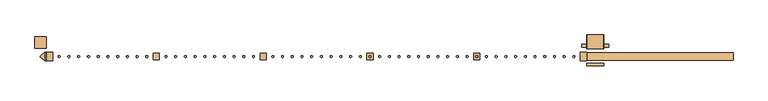
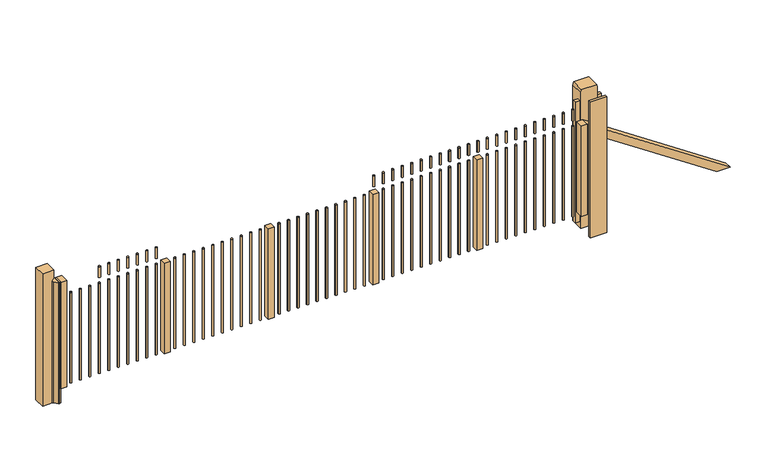
"""IFC4 building model written with IfcOpenShell, lengths in millimetres: door geometry, NLRS_90_DO_UN_schuifpoort met spijlen_gen_rsf : schuifpoort automatisch bxh 7000x1800-NP."""

from ifc_helpers import new_model, si_unit, point, frame, frame_2d, origin, place, context, project, spatial, polyline, circle_curve, trimmed, segment, composite_curve, outline, extrude, source, transform, mapped, element, save


def door_7189267d(model_context):
    return source(origin(), model_context, "Body", "SweptSolid", [
        extrude(outline(composite_curve([segment(trimmed(circle_curve(frame_2d((3299.5, 0.0)), 12.5), [point((3312.0, 0.0))], [point((3287.0, 0.0))], False, "CARTESIAN"), True, "CONTINUOUS"), segment(trimmed(circle_curve(frame_2d((3299.5, 0.0)), 12.5), [point((3287.0, 0.0))], [point((3312.0, 0.0))], False, "CARTESIAN"), True, "CONTINUOUS")], self_intersect=False)), frame((0.0, 0.0, 300.0), z_axis=(0.0, 0.0, 1.0), x_axis=(1.0, 0.0, 0.0)), (0.0, 0.0, 1.0), 1270.0),
        extrude(outline(composite_curve([segment(trimmed(circle_curve(frame_2d((3173.5, 0.0)), 12.5), [point((3186.0, 0.0))], [point((3161.0, 0.0))], False, "CARTESIAN"), True, "CONTINUOUS"), segment(trimmed(circle_curve(frame_2d((3173.5, 0.0)), 12.5), [point((3161.0, 0.0))], [point((3186.0, 0.0))], False, "CARTESIAN"), True, "CONTINUOUS")], self_intersect=False)), frame((0.0, 0.0, 300.0), z_axis=(0.0, 0.0, 1.0), x_axis=(1.0, 0.0, 0.0)), (0.0, 0.0, 1.0), 1270.0),
        extrude(outline(composite_curve([segment(trimmed(circle_curve(frame_2d((3047.5, 0.0)), 12.5), [point((3060.0, 0.0))], [point((3035.0, 0.0))], False, "CARTESIAN"), True, "CONTINUOUS"), segment(trimmed(circle_curve(frame_2d((3047.5, 0.0)), 12.5), [point((3035.0, 0.0))], [point((3060.0, 0.0))], False, "CARTESIAN"), True, "CONTINUOUS")], self_intersect=False)), frame((0.0, 0.0, 300.0), z_axis=(0.0, 0.0, 1.0), x_axis=(1.0, 0.0, 0.0)), (0.0, 0.0, 1.0), 1270.0),
        extrude(outline(composite_curve([segment(trimmed(circle_curve(frame_2d((2921.5, 0.0)), 12.5), [point((2934.0, 0.0))], [point((2909.0, 0.0))], False, "CARTESIAN"), True, "CONTINUOUS"), segment(trimmed(circle_curve(frame_2d((2921.5, 0.0)), 12.5), [point((2909.0, 0.0))], [point((2934.0, 0.0))], False, "CARTESIAN"), True, "CONTINUOUS")], self_intersect=False)), frame((0.0, 0.0, 300.0), z_axis=(0.0, 0.0, 1.0), x_axis=(1.0, 0.0, 0.0)), (0.0, 0.0, 1.0), 1270.0),
        extrude(outline(composite_curve([segment(trimmed(circle_curve(frame_2d((2795.5, 0.0)), 12.5), [point((2808.0, 0.0))], [point((2783.0, 0.0))], False, "CARTESIAN"), True, "CONTINUOUS"), segment(trimmed(circle_curve(frame_2d((2795.5, 0.0)), 12.5), [point((2783.0, 0.0))], [point((2808.0, 0.0))], False, "CARTESIAN"), True, "CONTINUOUS")], self_intersect=False)), frame((0.0, 0.0, 300.0), z_axis=(0.0, 0.0, 1.0), x_axis=(1.0, 0.0, 0.0)), (0.0, 0.0, 1.0), 1270.0),
        extrude(outline(composite_curve([segment(trimmed(circle_curve(frame_2d((2669.5, 0.0)), 12.5), [point((2682.0, 0.0))], [point((2657.0, 0.0))], False, "CARTESIAN"), True, "CONTINUOUS"), segment(trimmed(circle_curve(frame_2d((2669.5, 0.0)), 12.5), [point((2657.0, 0.0))], [point((2682.0, 0.0))], False, "CARTESIAN"), True, "CONTINUOUS")], self_intersect=False)), frame((0.0, 0.0, 300.0), z_axis=(0.0, 0.0, 1.0), x_axis=(1.0, 0.0, 0.0)), (0.0, 0.0, 1.0), 1270.0),
        extrude(outline(composite_curve([segment(trimmed(circle_curve(frame_2d((2543.5, 0.0)), 12.5), [point((2556.0, 0.0))], [point((2531.0, 0.0))], False, "CARTESIAN"), True, "CONTINUOUS"), segment(trimmed(circle_curve(frame_2d((2543.5, 0.0)), 12.5), [point((2531.0, 0.0))], [point((2556.0, 0.0))], False, "CARTESIAN"), True, "CONTINUOUS")], self_intersect=False)), frame((0.0, 0.0, 300.0), z_axis=(0.0, 0.0, 1.0), x_axis=(1.0, 0.0, 0.0)), (0.0, 0.0, 1.0), 1270.0),
        extrude(outline(composite_curve([segment(trimmed(circle_curve(frame_2d((2417.5, 0.0)), 12.5), [point((2430.0, 0.0))], [point((2405.0, 0.0))], False, "CARTESIAN"), True, "CONTINUOUS"), segment(trimmed(circle_curve(frame_2d((2417.5, 0.0)), 12.5), [point((2405.0, 0.0))], [point((2430.0, 0.0))], False, "CARTESIAN"), True, "CONTINUOUS")], self_intersect=False)), frame((0.0, 0.0, 300.0), z_axis=(0.0, 0.0, 1.0), x_axis=(1.0, 0.0, 0.0)), (0.0, 0.0, 1.0), 1270.0),
        extrude(outline(composite_curve([segment(trimmed(circle_curve(frame_2d((2291.5, 0.0)), 12.5), [point((2304.0, 0.0))], [point((2279.0, 0.0))], False, "CARTESIAN"), True, "CONTINUOUS"), segment(trimmed(circle_curve(frame_2d((2291.5, 0.0)), 12.5), [point((2279.0, 0.0))], [point((2304.0, 0.0))], False, "CARTESIAN"), True, "CONTINUOUS")], self_intersect=False)), frame((0.0, 0.0, 300.0), z_axis=(0.0, 0.0, 1.0), x_axis=(1.0, 0.0, 0.0)), (0.0, 0.0, 1.0), 1270.0),
        extrude(outline(composite_curve([segment(trimmed(circle_curve(frame_2d((2165.5, 0.0)), 12.5), [point((2178.0, 0.0))], [point((2153.0, 0.0))], False, "CARTESIAN"), True, "CONTINUOUS"), segment(trimmed(circle_curve(frame_2d((2165.5, 0.0)), 12.5), [point((2153.0, 0.0))], [point((2178.0, 0.0))], False, "CARTESIAN"), True, "CONTINUOUS")], self_intersect=False)), frame((0.0, 0.0, 300.0), z_axis=(0.0, 0.0, 1.0), x_axis=(1.0, 0.0, 0.0)), (0.0, 0.0, 1.0), 1270.0),
        extrude(outline(composite_curve([segment(trimmed(circle_curve(frame_2d((1915.5, 0.0)), 12.5), [point((1928.0, 0.0))], [point((1903.0, 0.0))], False, "CARTESIAN"), True, "CONTINUOUS"), segment(trimmed(circle_curve(frame_2d((1915.5, 0.0)), 12.5), [point((1903.0, 0.0))], [point((1928.0, 0.0))], False, "CARTESIAN"), True, "CONTINUOUS")], self_intersect=False)), frame((0.0, 0.0, 300.0), z_axis=(0.0, 0.0, 1.0), x_axis=(1.0, 0.0, 0.0)), (0.0, 0.0, 1.0), 1270.0),
        extrude(outline(composite_curve([segment(trimmed(circle_curve(frame_2d((1789.5, 0.0)), 12.5), [point((1802.0, 0.0))], [point((1777.0, 0.0))], False, "CARTESIAN"), True, "CONTINUOUS"), segment(trimmed(circle_curve(frame_2d((1789.5, 0.0)), 12.5), [point((1777.0, 0.0))], [point((1802.0, 0.0))], False, "CARTESIAN"), True, "CONTINUOUS")], self_intersect=False)), frame((0.0, 0.0, 300.0), z_axis=(0.0, 0.0, 1.0), x_axis=(1.0, 0.0, 0.0)), (0.0, 0.0, 1.0), 1270.0),
        extrude(outline(composite_curve([segment(trimmed(circle_curve(frame_2d((1663.5, 0.0)), 12.5), [point((1676.0, 0.0))], [point((1651.0, 0.0))], False, "CARTESIAN"), True, "CONTINUOUS"), segment(trimmed(circle_curve(frame_2d((1663.5, 0.0)), 12.5), [point((1651.0, 0.0))], [point((1676.0, 0.0))], False, "CARTESIAN"), True, "CONTINUOUS")], self_intersect=False)), frame((0.0, 0.0, 300.0), z_axis=(0.0, 0.0, 1.0), x_axis=(1.0, 0.0, 0.0)), (0.0, 0.0, 1.0), 1270.0),
        extrude(outline(composite_curve([segment(trimmed(circle_curve(frame_2d((1537.5, 0.0)), 12.5), [point((1550.0, 0.0))], [point((1525.0, 0.0))], False, "CARTESIAN"), True, "CONTINUOUS"), segment(trimmed(circle_curve(frame_2d((1537.5, 0.0)), 12.5), [point((1525.0, 0.0))], [point((1550.0, 0.0))], False, "CARTESIAN"), True, "CONTINUOUS")], self_intersect=False)), frame((0.0, 0.0, 300.0), z_axis=(0.0, 0.0, 1.0), x_axis=(1.0, 0.0, 0.0)), (0.0, 0.0, 1.0), 1270.0),
        extrude(outline(composite_curve([segment(trimmed(circle_curve(frame_2d((1411.5, 0.0)), 12.5), [point((1424.0, 0.0))], [point((1399.0, 0.0))], False, "CARTESIAN"), True, "CONTINUOUS"), segment(trimmed(circle_curve(frame_2d((1411.5, 0.0)), 12.5), [point((1399.0, 0.0))], [point((1424.0, 0.0))], False, "CARTESIAN"), True, "CONTINUOUS")], self_intersect=False)), frame((0.0, 0.0, 300.0), z_axis=(0.0, 0.0, 1.0), x_axis=(1.0, 0.0, 0.0)), (0.0, 0.0, 1.0), 1270.0),
        extrude(outline(composite_curve([segment(trimmed(circle_curve(frame_2d((1285.5, 0.0)), 12.5), [point((1298.0, 0.0))], [point((1273.0, 0.0))], False, "CARTESIAN"), True, "CONTINUOUS"), segment(trimmed(circle_curve(frame_2d((1285.5, 0.0)), 12.5), [point((1273.0, 0.0))], [point((1298.0, 0.0))], False, "CARTESIAN"), True, "CONTINUOUS")], self_intersect=False)), frame((0.0, 0.0, 300.0), z_axis=(0.0, 0.0, 1.0), x_axis=(1.0, 0.0, 0.0)), (0.0, 0.0, 1.0), 1270.0),
        extrude(outline(composite_curve([segment(trimmed(circle_curve(frame_2d((1159.5, 0.0)), 12.5), [point((1172.0, 0.0))], [point((1147.0, 0.0))], False, "CARTESIAN"), True, "CONTINUOUS"), segment(trimmed(circle_curve(frame_2d((1159.5, 0.0)), 12.5), [point((1147.0, 0.0))], [point((1172.0, 0.0))], False, "CARTESIAN"), True, "CONTINUOUS")], self_intersect=False)), frame((0.0, 0.0, 300.0), z_axis=(0.0, 0.0, 1.0), x_axis=(1.0, 0.0, 0.0)), (0.0, 0.0, 1.0), 1270.0),
        extrude(outline(composite_curve([segment(trimmed(circle_curve(frame_2d((1033.5, 0.0)), 12.5), [point((1046.0, 0.0))], [point((1021.0, 0.0))], False, "CARTESIAN"), True, "CONTINUOUS"), segment(trimmed(circle_curve(frame_2d((1033.5, 0.0)), 12.5), [point((1021.0, 0.0))], [point((1046.0, 0.0))], False, "CARTESIAN"), True, "CONTINUOUS")], self_intersect=False)), frame((0.0, 0.0, 300.0), z_axis=(0.0, 0.0, 1.0), x_axis=(1.0, 0.0, 0.0)), (0.0, 0.0, 1.0), 1270.0),
        extrude(outline(composite_curve([segment(trimmed(circle_curve(frame_2d((907.5, 0.0)), 12.5), [point((920.0, 0.0))], [point((895.0, 0.0))], False, "CARTESIAN"), True, "CONTINUOUS"), segment(trimmed(circle_curve(frame_2d((907.5, 0.0)), 12.5), [point((895.0, 0.0))], [point((920.0, 0.0))], False, "CARTESIAN"), True, "CONTINUOUS")], self_intersect=False)), frame((0.0, 0.0, 300.0), z_axis=(0.0, 0.0, 1.0), x_axis=(1.0, 0.0, 0.0)), (0.0, 0.0, 1.0), 1270.0),
        extrude(outline(composite_curve([segment(trimmed(circle_curve(frame_2d((781.5, 0.0)), 12.5), [point((794.0, 0.0))], [point((769.0, 0.0))], False, "CARTESIAN"), True, "CONTINUOUS"), segment(trimmed(circle_curve(frame_2d((781.5, 0.0)), 12.5), [point((769.0, 0.0))], [point((794.0, 0.0))], False, "CARTESIAN"), True, "CONTINUOUS")], self_intersect=False)), frame((0.0, 0.0, 300.0), z_axis=(0.0, 0.0, 1.0), x_axis=(1.0, 0.0, 0.0)), (0.0, 0.0, 1.0), 1270.0),
        extrude(outline(polyline([(3465.0, 158.5), (3465.0, 118.5), (3400.0, 118.5), (3400.0, 158.5), (3465.0, 158.5)])), frame((0.0, 0.0, 100.0), z_axis=(0.0, 0.0, 1.0), x_axis=(1.0, 0.0, 0.0)), (0.0, 0.0, 1.0), 1700.0),
        extrude(outline(polyline([(3685.0, 158.5), (3750.0, 158.5), (3750.0, 118.5), (3685.0, 118.5), (3685.0, 158.5)])), frame((0.0, 0.0, 100.0), z_axis=(0.0, 0.0, 1.0), x_axis=(1.0, 0.0, 0.0)), (0.0, 0.0, 1.0), 1700.0),
        extrude(outline(polyline([(3685.0, -84.5), (3685.0, -119.5), (3465.0, -119.5), (3465.0, -84.5), (3685.0, -84.5)])), frame((0.0, 0.0, 12.0), z_axis=(0.0, 0.0, 1.0), x_axis=(1.0, 0.0, 0.0)), (0.0, 0.0, 1.0), 1906.0),
        extrude(outline(polyline([(1918.0, 3465.0), (12.0, 3465.0), (12.0, 3685.0), (1918.0, 3685.0), (1960.0, 3677.5), (1960.0, 3472.5), (1918.0, 3465.0)])), frame((0.0, 100.5, 0.0), z_axis=(0.0, 1.0, 0.0), x_axis=(0.0, 0.0, 1.0)), (0.0, 0.0, 1.0), 180.0),
        extrude(outline(polyline([(2000.5, 40.0), (2080.5, 40.0), (2080.5, -40.0), (2000.5, -40.0), (2000.5, 40.0)])), frame((0.0, 0.0, 300.0), z_axis=(0.0, 0.0, 1.0), x_axis=(1.0, 0.0, 0.0)), (0.0, 0.0, 1.0), 1270.0),
        extrude(outline(polyline([(616.5, 40.0), (696.5, 40.0), (696.5, -40.0), (616.5, -40.0), (616.5, 40.0)])), frame((0.0, 0.0, 300.0), z_axis=(0.0, 0.0, 1.0), x_axis=(1.0, 0.0, 0.0)), (0.0, 0.0, 1.0), 1270.0),
        extrude(outline(polyline([(-767.5, 40.0), (-687.5, 40.0), (-687.5, -40.0), (-767.5, -40.0), (-767.5, 40.0)])), frame((0.0, 0.0, 300.0), z_axis=(0.0, 0.0, 1.0), x_axis=(1.0, 0.0, 0.0)), (0.0, 0.0, 1.0), 1270.0),
        extrude(outline(polyline([(-2151.5, 40.0), (-2071.5, 40.0), (-2071.5, -40.0), (-2151.5, -40.0), (-2151.5, 40.0)])), frame((0.0, 0.0, 300.0), z_axis=(0.0, 0.0, 1.0), x_axis=(1.0, 0.0, 0.0)), (0.0, 0.0, 1.0), 1270.0),
        extrude(outline(composite_curve([segment(trimmed(circle_curve(frame_2d((531.5, 0.0)), 12.5), [point((544.0, 0.0))], [point((519.0, 0.0))], False, "CARTESIAN"), True, "CONTINUOUS"), segment(trimmed(circle_curve(frame_2d((531.5, 0.0)), 12.5), [point((519.0, 0.0))], [point((544.0, 0.0))], False, "CARTESIAN"), True, "CONTINUOUS")], self_intersect=False)), frame((0.0, 0.0, 300.0), z_axis=(0.0, 0.0, 1.0), x_axis=(1.0, 0.0, 0.0)), (0.0, 0.0, 1.0), 1270.0),
        extrude(outline(composite_curve([segment(trimmed(circle_curve(frame_2d((405.5, 0.0)), 12.5), [point((418.0, 0.0))], [point((393.0, 0.0))], False, "CARTESIAN"), True, "CONTINUOUS"), segment(trimmed(circle_curve(frame_2d((405.5, 0.0)), 12.5), [point((393.0, 0.0))], [point((418.0, 0.0))], False, "CARTESIAN"), True, "CONTINUOUS")], self_intersect=False)), frame((0.0, 0.0, 300.0), z_axis=(0.0, 0.0, 1.0), x_axis=(1.0, 0.0, 0.0)), (0.0, 0.0, 1.0), 1270.0),
        extrude(outline(composite_curve([segment(trimmed(circle_curve(frame_2d((279.5, 0.0)), 12.5), [point((292.0, 0.0))], [point((267.0, 0.0))], False, "CARTESIAN"), True, "CONTINUOUS"), segment(trimmed(circle_curve(frame_2d((279.5, 0.0)), 12.5), [point((267.0, 0.0))], [point((292.0, 0.0))], False, "CARTESIAN"), True, "CONTINUOUS")], self_intersect=False)), frame((0.0, 0.0, 300.0), z_axis=(0.0, 0.0, 1.0), x_axis=(1.0, 0.0, 0.0)), (0.0, 0.0, 1.0), 1270.0),
        extrude(outline(composite_curve([segment(trimmed(circle_curve(frame_2d((153.5, 0.0)), 12.5), [point((166.0, 0.0))], [point((141.0, 0.0))], False, "CARTESIAN"), True, "CONTINUOUS"), segment(trimmed(circle_curve(frame_2d((153.5, 0.0)), 12.5), [point((141.0, 0.0))], [point((166.0, 0.0))], False, "CARTESIAN"), True, "CONTINUOUS")], self_intersect=False)), frame((0.0, 0.0, 300.0), z_axis=(0.0, 0.0, 1.0), x_axis=(1.0, 0.0, 0.0)), (0.0, 0.0, 1.0), 1270.0),
        extrude(outline(composite_curve([segment(trimmed(circle_curve(frame_2d((27.5, 0.0)), 12.5), [point((40.0, 0.0))], [point((15.0, 0.0))], False, "CARTESIAN"), True, "CONTINUOUS"), segment(trimmed(circle_curve(frame_2d((27.5, 0.0)), 12.5), [point((15.0, 0.0))], [point((40.0, 0.0))], False, "CARTESIAN"), True, "CONTINUOUS")], self_intersect=False)), frame((0.0, 0.0, 300.0), z_axis=(0.0, 0.0, 1.0), x_axis=(1.0, 0.0, 0.0)), (0.0, 0.0, 1.0), 1270.0),
        extrude(outline(composite_curve([segment(trimmed(circle_curve(frame_2d((-98.5, 0.0)), 12.5), [point((-86.0, 0.0))], [point((-111.0, 0.0))], False, "CARTESIAN"), True, "CONTINUOUS"), segment(trimmed(circle_curve(frame_2d((-98.5, 0.0)), 12.5), [point((-111.0, 0.0))], [point((-86.0, 0.0))], False, "CARTESIAN"), True, "CONTINUOUS")], self_intersect=False)), frame((0.0, 0.0, 300.0), z_axis=(0.0, 0.0, 1.0), x_axis=(1.0, 0.0, 0.0)), (0.0, 0.0, 1.0), 1270.0),
        extrude(outline(composite_curve([segment(trimmed(circle_curve(frame_2d((-224.5, 0.0)), 12.5), [point((-212.0, 0.0))], [point((-237.0, 0.0))], False, "CARTESIAN"), True, "CONTINUOUS"), segment(trimmed(circle_curve(frame_2d((-224.5, 0.0)), 12.5), [point((-237.0, 0.0))], [point((-212.0, 0.0))], False, "CARTESIAN"), True, "CONTINUOUS")], self_intersect=False)), frame((0.0, 0.0, 300.0), z_axis=(0.0, 0.0, 1.0), x_axis=(1.0, 0.0, 0.0)), (0.0, 0.0, 1.0), 1270.0),
        extrude(outline(composite_curve([segment(trimmed(circle_curve(frame_2d((-350.5, 0.0)), 12.5), [point((-338.0, 0.0))], [point((-363.0, 0.0))], False, "CARTESIAN"), True, "CONTINUOUS"), segment(trimmed(circle_curve(frame_2d((-350.5, 0.0)), 12.5), [point((-363.0, 0.0))], [point((-338.0, 0.0))], False, "CARTESIAN"), True, "CONTINUOUS")], self_intersect=False)), frame((0.0, 0.0, 300.0), z_axis=(0.0, 0.0, 1.0), x_axis=(1.0, 0.0, 0.0)), (0.0, 0.0, 1.0), 1270.0),
        extrude(outline(composite_curve([segment(trimmed(circle_curve(frame_2d((-476.5, 0.0)), 12.5), [point((-464.0, 0.0))], [point((-489.0, 0.0))], False, "CARTESIAN"), True, "CONTINUOUS"), segment(trimmed(circle_curve(frame_2d((-476.5, 0.0)), 12.5), [point((-489.0, 0.0))], [point((-464.0, 0.0))], False, "CARTESIAN"), True, "CONTINUOUS")], self_intersect=False)), frame((0.0, 0.0, 300.0), z_axis=(0.0, 0.0, 1.0), x_axis=(1.0, 0.0, 0.0)), (0.0, 0.0, 1.0), 1270.0),
        extrude(outline(composite_curve([segment(trimmed(circle_curve(frame_2d((-602.5, 0.0)), 12.5), [point((-590.0, 0.0))], [point((-615.0, 0.0))], False, "CARTESIAN"), True, "CONTINUOUS"), segment(trimmed(circle_curve(frame_2d((-602.5, 0.0)), 12.5), [point((-615.0, 0.0))], [point((-590.0, 0.0))], False, "CARTESIAN"), True, "CONTINUOUS")], self_intersect=False)), frame((0.0, 0.0, 300.0), z_axis=(0.0, 0.0, 1.0), x_axis=(1.0, 0.0, 0.0)), (0.0, 0.0, 1.0), 1270.0),
        extrude(outline(polyline([(300.0, 5362.0), (1570.0, 3464.5), (1449.6685917, 3464.5), (300.0, 5182.2135061), (300.0, 5362.0)])), frame((0.0, -50.0, 0.0), z_axis=(0.0, 1.0, 0.0), x_axis=(0.0, 0.0, 1.0)), (0.0, 0.0, 1.0), 100.0),
        extrude(outline(composite_curve([segment(trimmed(circle_curve(frame_2d((-852.5, 0.0)), 12.5), [point((-840.0, 0.0))], [point((-865.0, 0.0))], False, "CARTESIAN"), True, "CONTINUOUS"), segment(trimmed(circle_curve(frame_2d((-852.5, 0.0)), 12.5), [point((-865.0, 0.0))], [point((-840.0, 0.0))], False, "CARTESIAN"), True, "CONTINUOUS")], self_intersect=False)), frame((0.0, 0.0, 300.0), z_axis=(0.0, 0.0, 1.0), x_axis=(1.0, 0.0, 0.0)), (0.0, 0.0, 1.0), 1270.0),
        extrude(outline(composite_curve([segment(trimmed(circle_curve(frame_2d((-978.5, 0.0)), 12.5), [point((-966.0, 0.0))], [point((-991.0, 0.0))], False, "CARTESIAN"), True, "CONTINUOUS"), segment(trimmed(circle_curve(frame_2d((-978.5, 0.0)), 12.5), [point((-991.0, 0.0))], [point((-966.0, 0.0))], False, "CARTESIAN"), True, "CONTINUOUS")], self_intersect=False)), frame((0.0, 0.0, 300.0), z_axis=(0.0, 0.0, 1.0), x_axis=(1.0, 0.0, 0.0)), (0.0, 0.0, 1.0), 1270.0),
        extrude(outline(composite_curve([segment(trimmed(circle_curve(frame_2d((-1104.5, 0.0)), 12.5), [point((-1092.0, 0.0))], [point((-1117.0, 0.0))], False, "CARTESIAN"), True, "CONTINUOUS"), segment(trimmed(circle_curve(frame_2d((-1104.5, 0.0)), 12.5), [point((-1117.0, 0.0))], [point((-1092.0, 0.0))], False, "CARTESIAN"), True, "CONTINUOUS")], self_intersect=False)), frame((0.0, 0.0, 300.0), z_axis=(0.0, 0.0, 1.0), x_axis=(1.0, 0.0, 0.0)), (0.0, 0.0, 1.0), 1270.0),
        extrude(outline(composite_curve([segment(trimmed(circle_curve(frame_2d((-1230.5, 0.0)), 12.5), [point((-1218.0, 0.0))], [point((-1243.0, 0.0))], False, "CARTESIAN"), True, "CONTINUOUS"), segment(trimmed(circle_curve(frame_2d((-1230.5, 0.0)), 12.5), [point((-1243.0, 0.0))], [point((-1218.0, 0.0))], False, "CARTESIAN"), True, "CONTINUOUS")], self_intersect=False)), frame((0.0, 0.0, 300.0), z_axis=(0.0, 0.0, 1.0), x_axis=(1.0, 0.0, 0.0)), (0.0, 0.0, 1.0), 1270.0),
        extrude(outline(composite_curve([segment(trimmed(circle_curve(frame_2d((-1356.5, 0.0)), 12.5), [point((-1344.0, 0.0))], [point((-1369.0, 0.0))], False, "CARTESIAN"), True, "CONTINUOUS"), segment(trimmed(circle_curve(frame_2d((-1356.5, 0.0)), 12.5), [point((-1369.0, 0.0))], [point((-1344.0, 0.0))], False, "CARTESIAN"), True, "CONTINUOUS")], self_intersect=False)), frame((0.0, 0.0, 300.0), z_axis=(0.0, 0.0, 1.0), x_axis=(1.0, 0.0, 0.0)), (0.0, 0.0, 1.0), 1270.0),
        extrude(outline(composite_curve([segment(trimmed(circle_curve(frame_2d((-1482.5, 0.0)), 12.5), [point((-1470.0, 0.0))], [point((-1495.0, 0.0))], False, "CARTESIAN"), True, "CONTINUOUS"), segment(trimmed(circle_curve(frame_2d((-1482.5, 0.0)), 12.5), [point((-1495.0, 0.0))], [point((-1470.0, 0.0))], False, "CARTESIAN"), True, "CONTINUOUS")], self_intersect=False)), frame((0.0, 0.0, 300.0), z_axis=(0.0, 0.0, 1.0), x_axis=(1.0, 0.0, 0.0)), (0.0, 0.0, 1.0), 1270.0),
        extrude(outline(composite_curve([segment(trimmed(circle_curve(frame_2d((-1608.5, 0.0)), 12.5), [point((-1596.0, 0.0))], [point((-1621.0, 0.0))], False, "CARTESIAN"), True, "CONTINUOUS"), segment(trimmed(circle_curve(frame_2d((-1608.5, 0.0)), 12.5), [point((-1621.0, 0.0))], [point((-1596.0, 0.0))], False, "CARTESIAN"), True, "CONTINUOUS")], self_intersect=False)), frame((0.0, 0.0, 300.0), z_axis=(0.0, 0.0, 1.0), x_axis=(1.0, 0.0, 0.0)), (0.0, 0.0, 1.0), 1270.0),
        extrude(outline(composite_curve([segment(trimmed(circle_curve(frame_2d((-1734.5, 0.0)), 12.5), [point((-1722.0, 0.0))], [point((-1747.0, 0.0))], False, "CARTESIAN"), True, "CONTINUOUS"), segment(trimmed(circle_curve(frame_2d((-1734.5, 0.0)), 12.5), [point((-1747.0, 0.0))], [point((-1722.0, 0.0))], False, "CARTESIAN"), True, "CONTINUOUS")], self_intersect=False)), frame((0.0, 0.0, 300.0), z_axis=(0.0, 0.0, 1.0), x_axis=(1.0, 0.0, 0.0)), (0.0, 0.0, 1.0), 1270.0),
        extrude(outline(composite_curve([segment(trimmed(circle_curve(frame_2d((-1860.5, 0.0)), 12.5), [point((-1848.0, 0.0))], [point((-1873.0, 0.0))], False, "CARTESIAN"), True, "CONTINUOUS"), segment(trimmed(circle_curve(frame_2d((-1860.5, 0.0)), 12.5), [point((-1873.0, 0.0))], [point((-1848.0, 0.0))], False, "CARTESIAN"), True, "CONTINUOUS")], self_intersect=False)), frame((0.0, 0.0, 300.0), z_axis=(0.0, 0.0, 1.0), x_axis=(1.0, 0.0, 0.0)), (0.0, 0.0, 1.0), 1270.0),
        extrude(outline(composite_curve([segment(trimmed(circle_curve(frame_2d((-1986.5, 0.0)), 12.5), [point((-1974.0, 0.0))], [point((-1999.0, 0.0))], False, "CARTESIAN"), True, "CONTINUOUS"), segment(trimmed(circle_curve(frame_2d((-1986.5, 0.0)), 12.5), [point((-1999.0, 0.0))], [point((-1974.0, 0.0))], False, "CARTESIAN"), True, "CONTINUOUS")], self_intersect=False)), frame((0.0, 0.0, 300.0), z_axis=(0.0, 0.0, 1.0), x_axis=(1.0, 0.0, 0.0)), (0.0, 0.0, 1.0), 1270.0),
        extrude(outline(composite_curve([segment(trimmed(circle_curve(frame_2d((-2236.0, 0.0)), 12.5), [point((-2223.5, 0.0))], [point((-2248.5, 0.0))], False, "CARTESIAN"), True, "CONTINUOUS"), segment(trimmed(circle_curve(frame_2d((-2236.0, 0.0)), 12.5), [point((-2248.5, 0.0))], [point((-2223.5, 0.0))], False, "CARTESIAN"), True, "CONTINUOUS")], self_intersect=False)), frame((0.0, 0.0, 300.0), z_axis=(0.0, 0.0, 1.0), x_axis=(1.0, 0.0, 0.0)), (0.0, 0.0, 1.0), 1270.0),
        extrude(outline(composite_curve([segment(trimmed(circle_curve(frame_2d((-2362.0, 0.0)), 12.5), [point((-2349.5, 0.0))], [point((-2374.5, 0.0))], False, "CARTESIAN"), True, "CONTINUOUS"), segment(trimmed(circle_curve(frame_2d((-2362.0, 0.0)), 12.5), [point((-2374.5, 0.0))], [point((-2349.5, 0.0))], False, "CARTESIAN"), True, "CONTINUOUS")], self_intersect=False)), frame((0.0, 0.0, 300.0), z_axis=(0.0, 0.0, 1.0), x_axis=(1.0, 0.0, 0.0)), (0.0, 0.0, 1.0), 1270.0),
        extrude(outline(composite_curve([segment(trimmed(circle_curve(frame_2d((-2488.0, 0.0)), 12.5), [point((-2475.5, 0.0))], [point((-2500.5, 0.0))], False, "CARTESIAN"), True, "CONTINUOUS"), segment(trimmed(circle_curve(frame_2d((-2488.0, 0.0)), 12.5), [point((-2500.5, 0.0))], [point((-2475.5, 0.0))], False, "CARTESIAN"), True, "CONTINUOUS")], self_intersect=False)), frame((0.0, 0.0, 300.0), z_axis=(0.0, 0.0, 1.0), x_axis=(1.0, 0.0, 0.0)), (0.0, 0.0, 1.0), 1270.0),
        extrude(outline(composite_curve([segment(trimmed(circle_curve(frame_2d((-2614.0, 0.0)), 12.5), [point((-2601.5, 0.0))], [point((-2626.5, 0.0))], False, "CARTESIAN"), True, "CONTINUOUS"), segment(trimmed(circle_curve(frame_2d((-2614.0, 0.0)), 12.5), [point((-2626.5, 0.0))], [point((-2601.5, 0.0))], False, "CARTESIAN"), True, "CONTINUOUS")], self_intersect=False)), frame((0.0, 0.0, 300.0), z_axis=(0.0, 0.0, 1.0), x_axis=(1.0, 0.0, 0.0)), (0.0, 0.0, 1.0), 1270.0),
        extrude(outline(composite_curve([segment(trimmed(circle_curve(frame_2d((-2740.0, 0.0)), 12.5), [point((-2727.5, 0.0))], [point((-2752.5, 0.0))], False, "CARTESIAN"), True, "CONTINUOUS"), segment(trimmed(circle_curve(frame_2d((-2740.0, 0.0)), 12.5), [point((-2752.5, 0.0))], [point((-2727.5, 0.0))], False, "CARTESIAN"), True, "CONTINUOUS")], self_intersect=False)), frame((0.0, 0.0, 300.0), z_axis=(0.0, 0.0, 1.0), x_axis=(1.0, 0.0, 0.0)), (0.0, 0.0, 1.0), 1270.0),
        extrude(outline(composite_curve([segment(trimmed(circle_curve(frame_2d((-2866.0, 0.0)), 12.5), [point((-2853.5, 0.0))], [point((-2878.5, 0.0))], False, "CARTESIAN"), True, "CONTINUOUS"), segment(trimmed(circle_curve(frame_2d((-2866.0, 0.0)), 12.5), [point((-2878.5, 0.0))], [point((-2853.5, 0.0))], False, "CARTESIAN"), True, "CONTINUOUS")], self_intersect=False)), frame((0.0, 0.0, 300.0), z_axis=(0.0, 0.0, 1.0), x_axis=(1.0, 0.0, 0.0)), (0.0, 0.0, 1.0), 1270.0),
        extrude(outline(composite_curve([segment(trimmed(circle_curve(frame_2d((-2992.0, 0.0)), 12.5), [point((-2979.5, 0.0))], [point((-3004.5, 0.0))], False, "CARTESIAN"), True, "CONTINUOUS"), segment(trimmed(circle_curve(frame_2d((-2992.0, 0.0)), 12.5), [point((-3004.5, 0.0))], [point((-2979.5, 0.0))], False, "CARTESIAN"), True, "CONTINUOUS")], self_intersect=False)), frame((0.0, 0.0, 300.0), z_axis=(0.0, 0.0, 1.0), x_axis=(1.0, 0.0, 0.0)), (0.0, 0.0, 1.0), 1270.0),
        extrude(outline(composite_curve([segment(trimmed(circle_curve(frame_2d((-3118.0, 0.0)), 12.5), [point((-3105.5, 0.0))], [point((-3130.5, 0.0))], False, "CARTESIAN"), True, "CONTINUOUS"), segment(trimmed(circle_curve(frame_2d((-3118.0, 0.0)), 12.5), [point((-3130.5, 0.0))], [point((-3105.5, 0.0))], False, "CARTESIAN"), True, "CONTINUOUS")], self_intersect=False)), frame((0.0, 0.0, 300.0), z_axis=(0.0, 0.0, 1.0), x_axis=(1.0, 0.0, 0.0)), (0.0, 0.0, 1.0), 1270.0),
        extrude(outline(composite_curve([segment(trimmed(circle_curve(frame_2d((-3244.0, 0.0)), 12.5), [point((-3231.5, 0.0))], [point((-3256.5, 0.0))], False, "CARTESIAN"), True, "CONTINUOUS"), segment(trimmed(circle_curve(frame_2d((-3244.0, 0.0)), 12.5), [point((-3256.5, 0.0))], [point((-3231.5, 0.0))], False, "CARTESIAN"), True, "CONTINUOUS")], self_intersect=False)), frame((0.0, 0.0, 300.0), z_axis=(0.0, 0.0, 1.0), x_axis=(1.0, 0.0, 0.0)), (0.0, 0.0, 1.0), 1270.0),
        extrude(outline(composite_curve([segment(trimmed(circle_curve(frame_2d((-3370.0, 0.0)), 12.5), [point((-3357.5, 0.0))], [point((-3382.5, 0.0))], False, "CARTESIAN"), True, "CONTINUOUS"), segment(trimmed(circle_curve(frame_2d((-3370.0, 0.0)), 12.5), [point((-3382.5, 0.0))], [point((-3357.5, 0.0))], False, "CARTESIAN"), True, "CONTINUOUS")], self_intersect=False)), frame((0.0, 0.0, 300.0), z_axis=(0.0, 0.0, 1.0), x_axis=(1.0, 0.0, 0.0)), (0.0, 0.0, 1.0), 1270.0),
        extrude(outline(composite_curve([segment(polyline([(-3558.78125, -54.1621094), (-3609.625, -11.4902343)]), True, "CONTINUOUS"), segment(trimmed(circle_curve(frame_2d((-3600.0040885, 0.0)), 14.9862412), [point((-3609.625, -11.4902343))], [point((-3609.625, 11.4902343))], False, "CARTESIAN"), True, "CONTINUOUS"), segment(polyline([(-3609.625, 11.4902343), (-3558.765625, 54.1777344)]), True, "CONTINUOUS"), segment(trimmed(circle_curve(frame_2d((-3557.4950392, 52.6395691)), 1.9950791), [point((-3558.765625, 54.1777344))], [point((-3555.53125, 52.2876138))], False, "CARTESIAN"), True, "CONTINUOUS"), segment(polyline([(-3555.53125, 52.2876138), (-3555.53125, -52.8919162)]), True, "CONTINUOUS"), segment(trimmed(circle_curve(frame_2d((-3557.5075149, -52.6282432)), 1.9937769), [point((-3555.53125, -52.8919162))], [point((-3558.78125, -54.1621094))], False, "CARTESIAN"), True, "CONTINUOUS")], self_intersect=False)), frame((0.0, 0.0, 100.0), z_axis=(0.0, 0.0, 1.0), x_axis=(1.0, 0.0, 0.0)), (0.0, 0.0, 1.0), 1700.0),
        extrude(outline(polyline([(-3535.5, 52.8125), (-3535.5, -52.8125), (-3555.53125, -52.8125), (-3555.53125, 52.8125), (-3535.5, 52.8125)])), frame((0.0, 0.0, 100.0), z_axis=(0.0, 0.0, 1.0), x_axis=(1.0, 0.0, 0.0)), (0.0, 0.0, 1.0), 1700.0),
        extrude(outline(polyline([(-3535.0, 255.5), (-3535.0, 105.5), (-3685.0, 105.5), (-3685.0, 255.5), (-3535.0, 255.5)])), frame((0.0, 0.0, 12.0), z_axis=(0.0, 0.0, 1.0), x_axis=(1.0, 0.0, 0.0)), (0.0, 0.0, 1.0), 1861.0),
        extrude(outline(polyline([(3464.5, 55.0), (3464.5, -55.0), (3384.5, -55.0), (3384.5, 55.0), (3464.5, 55.0)])), frame((0.0, 0.0, 300.0), z_axis=(0.0, 0.0, 1.0), x_axis=(1.0, 0.0, 0.0)), (0.0, 0.0, 1.0), 1270.0),
        extrude(outline(polyline([(-3455.5, 55.0), (-3455.5, -55.0), (-3535.5, -55.0), (-3535.5, 55.0), (-3455.5, 55.0)])), frame((0.0, 0.0, 300.0), z_axis=(0.0, 0.0, 1.0), x_axis=(1.0, 0.0, 0.0)), (0.0, 0.0, 1.0), 1500.0),
        extrude(outline(composite_curve([segment(trimmed(circle_curve(frame_2d((3299.5, 0.0)), 12.5), [point((3312.0, 0.0))], [point((3287.0, 0.0))], False, "CARTESIAN"), True, "CONTINUOUS"), segment(trimmed(circle_curve(frame_2d((3299.5, 0.0)), 12.5), [point((3287.0, 0.0))], [point((3312.0, 0.0))], False, "CARTESIAN"), True, "CONTINUOUS")], self_intersect=False)), frame((0.0, 0.0, 1650.0), z_axis=(0.0, 0.0, 1.0), x_axis=(1.0, 0.0, 0.0)), (0.0, 0.0, 1.0), 150.0),
        extrude(outline(composite_curve([segment(trimmed(circle_curve(frame_2d((3173.5, 0.0)), 12.5), [point((3186.0, 0.0))], [point((3161.0, 0.0))], False, "CARTESIAN"), True, "CONTINUOUS"), segment(trimmed(circle_curve(frame_2d((3173.5, 0.0)), 12.5), [point((3161.0, 0.0))], [point((3186.0, 0.0))], False, "CARTESIAN"), True, "CONTINUOUS")], self_intersect=False)), frame((0.0, 0.0, 1650.0), z_axis=(0.0, 0.0, 1.0), x_axis=(1.0, 0.0, 0.0)), (0.0, 0.0, 1.0), 150.0),
        extrude(outline(composite_curve([segment(trimmed(circle_curve(frame_2d((3047.5, 0.0)), 12.5), [point((3060.0, 0.0))], [point((3035.0, 0.0))], False, "CARTESIAN"), True, "CONTINUOUS"), segment(trimmed(circle_curve(frame_2d((3047.5, 0.0)), 12.5), [point((3035.0, 0.0))], [point((3060.0, 0.0))], False, "CARTESIAN"), True, "CONTINUOUS")], self_intersect=False)), frame((0.0, 0.0, 1650.0), z_axis=(0.0, 0.0, 1.0), x_axis=(1.0, 0.0, 0.0)), (0.0, 0.0, 1.0), 150.0),
        extrude(outline(composite_curve([segment(trimmed(circle_curve(frame_2d((2921.5, 0.0)), 12.5), [point((2934.0, 0.0))], [point((2909.0, 0.0))], False, "CARTESIAN"), True, "CONTINUOUS"), segment(trimmed(circle_curve(frame_2d((2921.5, 0.0)), 12.5), [point((2909.0, 0.0))], [point((2934.0, 0.0))], False, "CARTESIAN"), True, "CONTINUOUS")], self_intersect=False)), frame((0.0, 0.0, 1650.0), z_axis=(0.0, 0.0, 1.0), x_axis=(1.0, 0.0, 0.0)), (0.0, 0.0, 1.0), 150.0),
        extrude(outline(composite_curve([segment(trimmed(circle_curve(frame_2d((2795.5, 0.0)), 12.5), [point((2808.0, 0.0))], [point((2783.0, 0.0))], False, "CARTESIAN"), True, "CONTINUOUS"), segment(trimmed(circle_curve(frame_2d((2795.5, 0.0)), 12.5), [point((2783.0, 0.0))], [point((2808.0, 0.0))], False, "CARTESIAN"), True, "CONTINUOUS")], self_intersect=False)), frame((0.0, 0.0, 1650.0), z_axis=(0.0, 0.0, 1.0), x_axis=(1.0, 0.0, 0.0)), (0.0, 0.0, 1.0), 150.0),
        extrude(outline(composite_curve([segment(trimmed(circle_curve(frame_2d((2669.5, 0.0)), 12.5), [point((2682.0, 0.0))], [point((2657.0, 0.0))], False, "CARTESIAN"), True, "CONTINUOUS"), segment(trimmed(circle_curve(frame_2d((2669.5, 0.0)), 12.5), [point((2657.0, 0.0))], [point((2682.0, 0.0))], False, "CARTESIAN"), True, "CONTINUOUS")], self_intersect=False)), frame((0.0, 0.0, 1650.0), z_axis=(0.0, 0.0, 1.0), x_axis=(1.0, 0.0, 0.0)), (0.0, 0.0, 1.0), 150.0),
        extrude(outline(composite_curve([segment(trimmed(circle_curve(frame_2d((2543.5, 0.0)), 12.5), [point((2556.0, 0.0))], [point((2531.0, 0.0))], False, "CARTESIAN"), True, "CONTINUOUS"), segment(trimmed(circle_curve(frame_2d((2543.5, 0.0)), 12.5), [point((2531.0, 0.0))], [point((2556.0, 0.0))], False, "CARTESIAN"), True, "CONTINUOUS")], self_intersect=False)), frame((0.0, 0.0, 1650.0), z_axis=(0.0, 0.0, 1.0), x_axis=(1.0, 0.0, 0.0)), (0.0, 0.0, 1.0), 150.0),
        extrude(outline(composite_curve([segment(trimmed(circle_curve(frame_2d((2417.5, 0.0)), 12.5), [point((2430.0, 0.0))], [point((2405.0, 0.0))], False, "CARTESIAN"), True, "CONTINUOUS"), segment(trimmed(circle_curve(frame_2d((2417.5, 0.0)), 12.5), [point((2405.0, 0.0))], [point((2430.0, 0.0))], False, "CARTESIAN"), True, "CONTINUOUS")], self_intersect=False)), frame((0.0, 0.0, 1650.0), z_axis=(0.0, 0.0, 1.0), x_axis=(1.0, 0.0, 0.0)), (0.0, 0.0, 1.0), 150.0),
        extrude(outline(composite_curve([segment(trimmed(circle_curve(frame_2d((2291.5, 0.0)), 12.5), [point((2304.0, 0.0))], [point((2279.0, 0.0))], False, "CARTESIAN"), True, "CONTINUOUS"), segment(trimmed(circle_curve(frame_2d((2291.5, 0.0)), 12.5), [point((2279.0, 0.0))], [point((2304.0, 0.0))], False, "CARTESIAN"), True, "CONTINUOUS")], self_intersect=False)), frame((0.0, 0.0, 1650.0), z_axis=(0.0, 0.0, 1.0), x_axis=(1.0, 0.0, 0.0)), (0.0, 0.0, 1.0), 150.0),
        extrude(outline(composite_curve([segment(trimmed(circle_curve(frame_2d((2165.5, 0.0)), 12.5), [point((2178.0, 0.0))], [point((2153.0, 0.0))], False, "CARTESIAN"), True, "CONTINUOUS"), segment(trimmed(circle_curve(frame_2d((2165.5, 0.0)), 12.5), [point((2153.0, 0.0))], [point((2178.0, 0.0))], False, "CARTESIAN"), True, "CONTINUOUS")], self_intersect=False)), frame((0.0, 0.0, 1650.0), z_axis=(0.0, 0.0, 1.0), x_axis=(1.0, 0.0, 0.0)), (0.0, 0.0, 1.0), 150.0),
        extrude(outline(composite_curve([segment(trimmed(circle_curve(frame_2d((2040.5, 0.0)), 12.5), [point((2053.0, 0.0))], [point((2028.0, 0.0))], False, "CARTESIAN"), True, "CONTINUOUS"), segment(trimmed(circle_curve(frame_2d((2040.5, 0.0)), 12.5), [point((2028.0, 0.0))], [point((2053.0, 0.0))], False, "CARTESIAN"), True, "CONTINUOUS")], self_intersect=False)), frame((0.0, 0.0, 1650.0), z_axis=(0.0, 0.0, 1.0), x_axis=(1.0, 0.0, 0.0)), (0.0, 0.0, 1.0), 150.0),
        extrude(outline(composite_curve([segment(trimmed(circle_curve(frame_2d((656.5, 0.0)), 12.5), [point((669.0, 0.0))], [point((644.0, 0.0))], False, "CARTESIAN"), True, "CONTINUOUS"), segment(trimmed(circle_curve(frame_2d((656.5, 0.0)), 12.5), [point((644.0, 0.0))], [point((669.0, 0.0))], False, "CARTESIAN"), True, "CONTINUOUS")], self_intersect=False)), frame((0.0, 0.0, 1650.0), z_axis=(0.0, 0.0, 1.0), x_axis=(1.0, 0.0, 0.0)), (0.0, 0.0, 1.0), 150.0),
        extrude(outline(composite_curve([segment(trimmed(circle_curve(frame_2d((1915.5, 0.0)), 12.5), [point((1928.0, 0.0))], [point((1903.0, 0.0))], False, "CARTESIAN"), True, "CONTINUOUS"), segment(trimmed(circle_curve(frame_2d((1915.5, 0.0)), 12.5), [point((1903.0, 0.0))], [point((1928.0, 0.0))], False, "CARTESIAN"), True, "CONTINUOUS")], self_intersect=False)), frame((0.0, 0.0, 1650.0), z_axis=(0.0, 0.0, 1.0), x_axis=(1.0, 0.0, 0.0)), (0.0, 0.0, 1.0), 150.0),
        extrude(outline(composite_curve([segment(trimmed(circle_curve(frame_2d((1789.5, 0.0)), 12.5), [point((1802.0, 0.0))], [point((1777.0, 0.0))], False, "CARTESIAN"), True, "CONTINUOUS"), segment(trimmed(circle_curve(frame_2d((1789.5, 0.0)), 12.5), [point((1777.0, 0.0))], [point((1802.0, 0.0))], False, "CARTESIAN"), True, "CONTINUOUS")], self_intersect=False)), frame((0.0, 0.0, 1650.0), z_axis=(0.0, 0.0, 1.0), x_axis=(1.0, 0.0, 0.0)), (0.0, 0.0, 1.0), 150.0),
        extrude(outline(composite_curve([segment(trimmed(circle_curve(frame_2d((1663.5, 0.0)), 12.5), [point((1676.0, 0.0))], [point((1651.0, 0.0))], False, "CARTESIAN"), True, "CONTINUOUS"), segment(trimmed(circle_curve(frame_2d((1663.5, 0.0)), 12.5), [point((1651.0, 0.0))], [point((1676.0, 0.0))], False, "CARTESIAN"), True, "CONTINUOUS")], self_intersect=False)), frame((0.0, 0.0, 1650.0), z_axis=(0.0, 0.0, 1.0), x_axis=(1.0, 0.0, 0.0)), (0.0, 0.0, 1.0), 150.0),
        extrude(outline(composite_curve([segment(trimmed(circle_curve(frame_2d((1537.5, 0.0)), 12.5), [point((1550.0, 0.0))], [point((1525.0, 0.0))], False, "CARTESIAN"), True, "CONTINUOUS"), segment(trimmed(circle_curve(frame_2d((1537.5, 0.0)), 12.5), [point((1525.0, 0.0))], [point((1550.0, 0.0))], False, "CARTESIAN"), True, "CONTINUOUS")], self_intersect=False)), frame((0.0, 0.0, 1650.0), z_axis=(0.0, 0.0, 1.0), x_axis=(1.0, 0.0, 0.0)), (0.0, 0.0, 1.0), 150.0),
        extrude(outline(composite_curve([segment(trimmed(circle_curve(frame_2d((1411.5, 0.0)), 12.5), [point((1424.0, 0.0))], [point((1399.0, 0.0))], False, "CARTESIAN"), True, "CONTINUOUS"), segment(trimmed(circle_curve(frame_2d((1411.5, 0.0)), 12.5), [point((1399.0, 0.0))], [point((1424.0, 0.0))], False, "CARTESIAN"), True, "CONTINUOUS")], self_intersect=False)), frame((0.0, 0.0, 1650.0), z_axis=(0.0, 0.0, 1.0), x_axis=(1.0, 0.0, 0.0)), (0.0, 0.0, 1.0), 150.0),
        extrude(outline(composite_curve([segment(trimmed(circle_curve(frame_2d((1285.5, 0.0)), 12.5), [point((1298.0, 0.0))], [point((1273.0, 0.0))], False, "CARTESIAN"), True, "CONTINUOUS"), segment(trimmed(circle_curve(frame_2d((1285.5, 0.0)), 12.5), [point((1273.0, 0.0))], [point((1298.0, 0.0))], False, "CARTESIAN"), True, "CONTINUOUS")], self_intersect=False)), frame((0.0, 0.0, 1650.0), z_axis=(0.0, 0.0, 1.0), x_axis=(1.0, 0.0, 0.0)), (0.0, 0.0, 1.0), 150.0),
        extrude(outline(composite_curve([segment(trimmed(circle_curve(frame_2d((1159.5, 0.0)), 12.5), [point((1172.0, 0.0))], [point((1147.0, 0.0))], False, "CARTESIAN"), True, "CONTINUOUS"), segment(trimmed(circle_curve(frame_2d((1159.5, 0.0)), 12.5), [point((1147.0, 0.0))], [point((1172.0, 0.0))], False, "CARTESIAN"), True, "CONTINUOUS")], self_intersect=False)), frame((0.0, 0.0, 1650.0), z_axis=(0.0, 0.0, 1.0), x_axis=(1.0, 0.0, 0.0)), (0.0, 0.0, 1.0), 150.0),
        extrude(outline(composite_curve([segment(trimmed(circle_curve(frame_2d((1033.5, 0.0)), 12.5), [point((1046.0, 0.0))], [point((1021.0, 0.0))], False, "CARTESIAN"), True, "CONTINUOUS"), segment(trimmed(circle_curve(frame_2d((1033.5, 0.0)), 12.5), [point((1021.0, 0.0))], [point((1046.0, 0.0))], False, "CARTESIAN"), True, "CONTINUOUS")], self_intersect=False)), frame((0.0, 0.0, 1650.0), z_axis=(0.0, 0.0, 1.0), x_axis=(1.0, 0.0, 0.0)), (0.0, 0.0, 1.0), 150.0),
        extrude(outline(composite_curve([segment(trimmed(circle_curve(frame_2d((907.5, 0.0)), 12.5), [point((920.0, 0.0))], [point((895.0, 0.0))], False, "CARTESIAN"), True, "CONTINUOUS"), segment(trimmed(circle_curve(frame_2d((907.5, 0.0)), 12.5), [point((895.0, 0.0))], [point((920.0, 0.0))], False, "CARTESIAN"), True, "CONTINUOUS")], self_intersect=False)), frame((0.0, 0.0, 1650.0), z_axis=(0.0, 0.0, 1.0), x_axis=(1.0, 0.0, 0.0)), (0.0, 0.0, 1.0), 150.0),
        extrude(outline(composite_curve([segment(trimmed(circle_curve(frame_2d((781.5, 0.0)), 12.5), [point((794.0, 0.0))], [point((769.0, 0.0))], False, "CARTESIAN"), True, "CONTINUOUS"), segment(trimmed(circle_curve(frame_2d((781.5, 0.0)), 12.5), [point((769.0, 0.0))], [point((794.0, 0.0))], False, "CARTESIAN"), True, "CONTINUOUS")], self_intersect=False)), frame((0.0, 0.0, 1650.0), z_axis=(0.0, 0.0, 1.0), x_axis=(1.0, 0.0, 0.0)), (0.0, 0.0, 1.0), 150.0),
        extrude(outline(composite_curve([segment(trimmed(circle_curve(frame_2d((-2233.5, 0.0)), 12.5), [point((-2221.0, 0.0))], [point((-2246.0, 0.0))], False, "CARTESIAN"), True, "CONTINUOUS"), segment(trimmed(circle_curve(frame_2d((-2233.5, 0.0)), 12.5), [point((-2246.0, 0.0))], [point((-2221.0, 0.0))], False, "CARTESIAN"), True, "CONTINUOUS")], self_intersect=False)), frame((0.0, 0.0, 1650.0), z_axis=(0.0, 0.0, 1.0), x_axis=(1.0, 0.0, 0.0)), (0.0, 0.0, 1.0), 150.0),
        extrude(outline(composite_curve([segment(trimmed(circle_curve(frame_2d((-2359.5, 0.0)), 12.5), [point((-2347.0, 0.0))], [point((-2372.0, 0.0))], False, "CARTESIAN"), True, "CONTINUOUS"), segment(trimmed(circle_curve(frame_2d((-2359.5, 0.0)), 12.5), [point((-2372.0, 0.0))], [point((-2347.0, 0.0))], False, "CARTESIAN"), True, "CONTINUOUS")], self_intersect=False)), frame((0.0, 0.0, 1650.0), z_axis=(0.0, 0.0, 1.0), x_axis=(1.0, 0.0, 0.0)), (0.0, 0.0, 1.0), 150.0),
        extrude(outline(composite_curve([segment(trimmed(circle_curve(frame_2d((-2485.5, 0.0)), 12.5), [point((-2473.0, 0.0))], [point((-2498.0, 0.0))], False, "CARTESIAN"), True, "CONTINUOUS"), segment(trimmed(circle_curve(frame_2d((-2485.5, 0.0)), 12.5), [point((-2498.0, 0.0))], [point((-2473.0, 0.0))], False, "CARTESIAN"), True, "CONTINUOUS")], self_intersect=False)), frame((0.0, 0.0, 1650.0), z_axis=(0.0, 0.0, 1.0), x_axis=(1.0, 0.0, 0.0)), (0.0, 0.0, 1.0), 150.0),
        extrude(outline(composite_curve([segment(trimmed(circle_curve(frame_2d((-2611.5, 0.0)), 12.5), [point((-2599.0, 0.0))], [point((-2624.0, 0.0))], False, "CARTESIAN"), True, "CONTINUOUS"), segment(trimmed(circle_curve(frame_2d((-2611.5, 0.0)), 12.5), [point((-2624.0, 0.0))], [point((-2599.0, 0.0))], False, "CARTESIAN"), True, "CONTINUOUS")], self_intersect=False)), frame((0.0, 0.0, 1650.0), z_axis=(0.0, 0.0, 1.0), x_axis=(1.0, 0.0, 0.0)), (0.0, 0.0, 1.0), 150.0),
        extrude(outline(composite_curve([segment(trimmed(circle_curve(frame_2d((-2737.5, 0.0)), 12.5), [point((-2725.0, 0.0))], [point((-2750.0, 0.0))], False, "CARTESIAN"), True, "CONTINUOUS"), segment(trimmed(circle_curve(frame_2d((-2737.5, 0.0)), 12.5), [point((-2750.0, 0.0))], [point((-2725.0, 0.0))], False, "CARTESIAN"), True, "CONTINUOUS")], self_intersect=False)), frame((0.0, 0.0, 1650.0), z_axis=(0.0, 0.0, 1.0), x_axis=(1.0, 0.0, 0.0)), (0.0, 0.0, 1.0), 150.0),
        extrude(outline(composite_curve([segment(trimmed(circle_curve(frame_2d((-2863.5, 0.0)), 12.5), [point((-2851.0, 0.0))], [point((-2876.0, 0.0))], False, "CARTESIAN"), True, "CONTINUOUS"), segment(trimmed(circle_curve(frame_2d((-2863.5, 0.0)), 12.5), [point((-2876.0, 0.0))], [point((-2851.0, 0.0))], False, "CARTESIAN"), True, "CONTINUOUS")], self_intersect=False)), frame((0.0, 0.0, 1650.0), z_axis=(0.0, 0.0, 1.0), x_axis=(1.0, 0.0, 0.0)), (0.0, 0.0, 1.0), 150.0),
        extrude(outline(composite_curve([segment(trimmed(circle_curve(frame_2d((-2989.5, 0.0)), 12.5), [point((-2977.0, 0.0))], [point((-3002.0, 0.0))], False, "CARTESIAN"), True, "CONTINUOUS"), segment(trimmed(circle_curve(frame_2d((-2989.5, 0.0)), 12.5), [point((-3002.0, 0.0))], [point((-2977.0, 0.0))], False, "CARTESIAN"), True, "CONTINUOUS")], self_intersect=False)), frame((0.0, 0.0, 1650.0), z_axis=(0.0, 0.0, 1.0), x_axis=(1.0, 0.0, 0.0)), (0.0, 0.0, 1.0), 150.0),
    ])


if __name__ == "__main__":
    model = new_model("IFC4")
    model_context = context("Model", 3, world=origin())
    ifc_project = project(units=[si_unit("LENGTHUNIT", "METRE", prefix="MILLI")], contexts=[model_context])
    site = spatial("IfcSite", under=ifc_project)
    building = spatial("IfcBuilding", under=site)
    placement = place(None, origin())
    door_shape = door_7189267d(model_context)
    element("IfcDoor", 1, ObjectType="NLRS_90_DO_UN_schuifpoort met spijlen_gen_rsf : schuifpoort automatisch bxh 7000x1800-NP", at=placement, inside=building, context=model_context, shape_type="MappedRepresentation", body=[
        mapped(door_shape, transform((0.0, 0.0, 0.0), x_axis=(1.0, 0.0, 0.0), y_axis=(0.0, 1.0, 0.0), z_axis=(0.0, 0.0, 1.0))),
    ])
    save(model, "model.ifc")

# Revit data of these elements
# Type "NLRS_90_DO_UN_schuifpoort met spijlen_gen_rsf : schuifpoort automatisch bxh 7000x1800-NP"
#   Type IfcGUID = "1A81voHkv98RYujw6ZYnX6"
#   IfcName[Type] = "schuifpoort automatisch bxh 7000x1800-NP"
#   IfcDescription[Type] = "schuifpoort doorgang bxh 7000x1800mm"
#   IfcExportAs[Type] = "IfcDoorType"
#   IfcExportType[Type] = "GATE"
#   NLRS_C_revit_versie = ""
#   NLRS_C_omschrijving_03 [instance default] = "doorgangsmaat"
#   NLRS_C_omschrijving_02 [instance default] = "stootplaat"
#   NLRS_C_omschrijving_01 [instance default] = "rolpoort"
#   NLRS_C_content_versie = ""
#   NLRS_C_content_provider = ""
#   NLRS_C_content_handleiding = ""
#   NLRS_C_content_datum_uitgifte = ""
#   NLRS_C_content_datum_gewijzigd = ""
#   NLRS_C_content_creator = ""
#   Model = "generiek"
#   Manufacturer = "Revit Standards Foundation"
#   Description = "schuifpoort doorgang bxh 7000x1800mm"
#   Assembly Code = "90.32"
#   NLRS_C_hoogte = 1800.00 mm
#   NLRS_C_breedte_03 = 7000.00 mm
#   NLRS_C_materiaal_02 = NLRS_n5_rubber_gen_bf
#   NLRS_C_materiaal_01 = NLRS_h4_aluminium 250-255-255_gen_rsf
#   URL = ""
#   Keynote = ""
#   Default Elevation = 0
# Element 1 (IfcDoor, "NLRS_90_DO_UN_schuifpoort met spijlen_gen_rsf : schuifpoort automatisch bxh 7000x1800-NP")
#   Materials on its faces: "NLRS_h4_aluminium 250-255-255_gen_rsf", "NLRS_n5_rubber_gen_bf"
# Materials
#   "NLRS_n5_rubber_gen_bf": class "N - Kunststoffen, rubbers", colour RGB 63 63 63, transparency 0, Keynote = "n5", Model = "generiek", Manufacturer = "Revit Standards Foundation", URL = "www.revitstandards.org", Description = "rubber daktegels 600x600mm", Cost = 0
#   "NLRS_h4_aluminium 250-255-255_gen_rsf": class "BCB class", colour RGB 250 255 255, transparency 0, Keynote = "h4", Model = "generiek", Manufacturer = "Revit Standards Foundation", URL = "www.revitstandards.org", Description = "aluminium wit", Cost = 0
